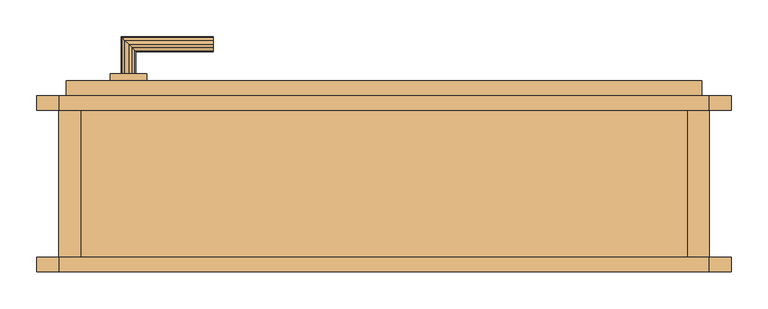
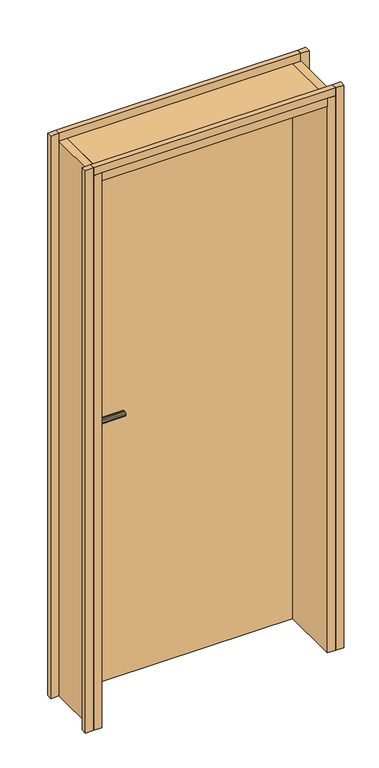
"""IFC4 building model written with IfcOpenShell, lengths in millimetres: door geometry, Tür."""

import ifcopenshell
import ifcopenshell.guid

model = None  # the IFC model being written
_history = None  # IfcOwnerHistory: only IFC2X3 demands one
_inside = {}  # id of a spatial element -> (the spatial element, [elements in it])
_under = {}  # id of a project, library or spatial element -> (it, [spatial elements below it])
_declared = {}  # id of a project -> (the project, [libraries it declares])
_typed = {}  # id of a type object -> (the type object, [elements of that type])
_made_of = {}  # id of a material, layer set ... -> (it, [elements and type objects made of it])


def new_model(schema):
    """Start an empty IFC model of exactly this schema.

    Asked for "IFC4X3", IfcOpenShell would pick the latest addendum, in which some entities
    have other attributes; the version numbers below select the first issue.
    IFC2X3 requires an IfcOwnerHistory on every rooted entity: one is made here for all.
    """
    global model, _history
    if schema == "IFC4X3":
        model = ifcopenshell.file(schema_version=(4, 3, 0, 0))
    else:
        model = ifcopenshell.file(schema=schema)
    _inside.clear()
    _under.clear()
    _declared.clear()
    _typed.clear()
    _made_of.clear()
    _history = None
    if model.schema == "IFC2X3":
        org = make("IfcOrganization", Name="unknown")
        user = make(
            "IfcPersonAndOrganization",
            ThePerson=make("IfcPerson", FamilyName="unknown"),
            TheOrganization=org,
        )
        app = make(
            "IfcApplication",
            ApplicationDeveloper=org,
            Version="unknown",
            ApplicationFullName="unknown",
            ApplicationIdentifier="unknown",
        )
        _history = make(
            "IfcOwnerHistory",
            OwningUser=user,
            OwningApplication=app,
            ChangeAction="ADDED",
            CreationDate=0,
        )
    return model


def make(cls, **values):
    """One entity of the class cls with the attributes given. An attribute that is None is left unset."""
    return model.create_entity(
        cls, **{name: value for name, value in values.items() if value is not None}
    )


def rooted(cls, **values):
    """An entity with a GlobalId (a new one), such as an element, a storey or a relation."""
    return make(cls, GlobalId=ifcopenshell.guid.new(), OwnerHistory=_history, **values)


def si_unit(unit_type, name, prefix=None):
    """IfcSIUnit, for example si_unit("LENGTHUNIT", "METRE", prefix="MILLI")."""
    return make("IfcSIUnit", UnitType=unit_type, Prefix=prefix, Name=name)


def assignment(units):
    """IfcUnitAssignment: the units of a project."""
    return None if units is None else make("IfcUnitAssignment", Units=units)


def point(xyz):
    """IfcCartesianPoint."""
    return None if xyz is None else make("IfcCartesianPoint", Coordinates=xyz)


def direction(xyz):
    """IfcDirection."""
    return None if xyz is None else make("IfcDirection", DirectionRatios=xyz)


def frame(location, z_axis=None, x_axis=None):
    """IfcAxis2Placement3D, a coordinate frame: its origin and axes. An axis left out is left unset."""
    return make(
        "IfcAxis2Placement3D",
        Location=point(location),
        Axis=direction(z_axis),
        RefDirection=direction(x_axis),
    )


def origin():
    """The frame at (0, 0, 0) with its axes left unset."""
    return frame((0.0, 0.0, 0.0))


def place(relative_to, where):
    """IfcLocalPlacement: puts the frame where relative to a parent placement (None: the world)."""
    return make(
        "IfcLocalPlacement", PlacementRelTo=relative_to, RelativePlacement=where
    )


def context(
    kind, dimensions, precision=None, world=None, true_north=None, identifier=None
):
    """IfcGeometricRepresentationContext, for example the 3D "Model" context."""
    return make(
        "IfcGeometricRepresentationContext",
        ContextIdentifier=identifier,
        ContextType=kind,
        CoordinateSpaceDimension=dimensions,
        Precision=precision,
        WorldCoordinateSystem=world,
        TrueNorth=true_north,
    )


def project(units=None, contexts=None):
    """IfcProject with its units and contexts."""
    return rooted(
        "IfcProject",
        Name="project",
        RepresentationContexts=contexts,
        UnitsInContext=assignment(units),
    )


def spatial(cls, under=None, at=None, **own):
    """A site, building, storey or space (cls), placed at a placement, below another one or the project."""
    s = rooted(cls, ObjectPlacement=at, **own)
    if under is not None:
        _under.setdefault(under.id(), (under, []))[1].append(s)
    return s


def polyline(points):
    """IfcPolyline through the points."""
    return make("IfcPolyline", Points=[point(p) for p in points])


def outline(outer, holes=None, kind="AREA"):
    """IfcArbitraryClosedProfileDef: a profile drawn as a closed curve; with holes, ...WithVoids."""
    if holes is None:
        return make("IfcArbitraryClosedProfileDef", ProfileType=kind, OuterCurve=outer)
    return make(
        "IfcArbitraryProfileDefWithVoids",
        ProfileType=kind,
        OuterCurve=outer,
        InnerCurves=holes,
    )


def extrude(swept, where, along, depth):
    """IfcExtrudedAreaSolid: the profile swept, set in the frame where, extruded along a direction by depth."""
    return make(
        "IfcExtrudedAreaSolid",
        SweptArea=swept,
        Position=where,
        ExtrudedDirection=direction(along),
        Depth=depth,
    )


def faces_of(points, faces, orient=None, outer=None):
    """IfcFace entities. A face is a list of loops; a loop is a list of indices into points, from 0.

    orient and outer hold one flag for each loop. By default every Orientation is true, the
    first loop of a face is its IfcFaceOuterBound and the others are IfcFaceBound.
    """
    made = []
    for i, loops in enumerate(faces):
        bounds = []
        for j, loop in enumerate(loops):
            is_outer = j == 0 if outer is None else outer[i][j]
            bounds.append(
                make(
                    "IfcFaceOuterBound" if is_outer else "IfcFaceBound",
                    Bound=make("IfcPolyLoop", Polygon=[points[k] for k in loop]),
                    Orientation=True if orient is None else orient[i][j],
                )
            )
        made.append(make("IfcFace", Bounds=bounds))
    return made


def faceted_brep(points, faces, orient=None, outer=None, voids=None):
    """IfcFacetedBrep: a solid bounded by flat faces; with voids (closed shells), ...WithVoids."""
    shared = [point(p) for p in points]
    hull = make("IfcClosedShell", CfsFaces=faces_of(shared, faces, orient, outer))
    if voids is None:
        return make("IfcFacetedBrep", Outer=hull)
    return make(
        "IfcFacetedBrepWithVoids",
        Outer=hull,
        Voids=[
            make(cls, CfsFaces=faces_of(shared, fs, o, b)) for cls, fs, o, b in voids
        ],
    )


def shape(context_of_items, identifier, shape_type, items):
    """IfcShapeRepresentation: the items that make up one representation, for example the "Body"."""
    return make(
        "IfcShapeRepresentation",
        ContextOfItems=context_of_items,
        RepresentationIdentifier=identifier,
        RepresentationType=shape_type,
        Items=items,
    )


def source(mapping_origin, context_of_items, identifier, shape_type, items):
    """IfcRepresentationMap: a shape defined once, which mapped items show again and again."""
    return make(
        "IfcRepresentationMap",
        MappingOrigin=mapping_origin,
        MappedRepresentation=shape(context_of_items, identifier, shape_type, items),
    )


def transform(
    local_origin,
    x_axis=None,
    y_axis=None,
    z_axis=None,
    scale=None,
    scale2=None,
    scale3=None,
    uniform=True,
):
    """IfcCartesianTransformationOperator3D, or its non-uniform kind. x_axis, y_axis, z_axis: its Axis1, 2, 3."""
    if uniform:
        return make(
            "IfcCartesianTransformationOperator3D",
            Axis1=direction(x_axis),
            Axis2=direction(y_axis),
            LocalOrigin=point(local_origin),
            Scale=scale,
            Axis3=direction(z_axis),
        )
    return make(
        "IfcCartesianTransformationOperator3DnonUniform",
        Axis1=direction(x_axis),
        Axis2=direction(y_axis),
        LocalOrigin=point(local_origin),
        Scale=scale,
        Axis3=direction(z_axis),
        Scale2=scale2,
        Scale3=scale3,
    )


def mapped(mapping_source, mapping_target):
    """IfcMappedItem: shows the shape of a source again, moved by a transform."""
    return make(
        "IfcMappedItem", MappingSource=mapping_source, MappingTarget=mapping_target
    )


def made_of(thing, what):
    """Note that an element or type object is made of a material, layer set ...; save() writes the relation."""
    if what is not None:
        _made_of.setdefault(what.id(), (what, []))[1].append(thing)
    return thing


def element(
    cls,
    number,
    at=None,
    inside=None,
    cuts=None,
    type_object=None,
    material=None,
    context=None,
    identifier="Body",
    shape_type=None,
    held_by="IfcProductDefinitionShape",
    body=None,
    shapes=None,
    **own,
):
    """One element of the class cls, such as IfcWall. Its Tag is "e" and its number.

    at: its placement. inside: the storey or other place that contains it. cuts: it is an
    opening in that element (IfcRelVoidsElement). A single representation is given by context,
    identifier, shape_type and body (its items); several are given by shapes. held_by: the class
    of the entity that holds the representations. save() writes the other relations.
    """
    e = rooted(cls, Tag="e%d" % number, ObjectPlacement=at, **own)
    if body is not None:
        shapes = [shape(context, identifier, shape_type, body)]
    if shapes is not None:
        e.Representation = make(held_by, Representations=shapes)
    if inside is not None:
        _inside.setdefault(inside.id(), (inside, []))[1].append(e)
    if cuts is not None:
        rooted(
            "IfcRelVoidsElement", RelatingBuildingElement=cuts, RelatedOpeningElement=e
        )
    if type_object is not None:
        _typed.setdefault(type_object.id(), (type_object, []))[1].append(e)
    return made_of(e, material)


def aggregate(whole, parts):
    """IfcRelAggregates: a whole, such as a stair, and the parts it consists of."""
    return rooted("IfcRelAggregates", RelatingObject=whole, RelatedObjects=parts)


def save(model, path):
    """Write the relations noted so far, then the file.

    IfcRelAggregates (storeys below a building ...), IfcRelContainedInSpatialStructure (elements
    in a storey), IfcRelDefinesByType, IfcRelAssociatesMaterial and IfcRelDeclares: one each for
    every whole, place, type object, material and project.
    """
    for whole, parts in _under.values():
        aggregate(whole, parts)
    for where, things in _inside.values():
        rooted(
            "IfcRelContainedInSpatialStructure",
            RelatedElements=things,
            RelatingStructure=where,
        )
    for kind, things in _typed.values():
        rooted("IfcRelDefinesByType", RelatedObjects=things, RelatingType=kind)
    for what, things in _made_of.values():
        rooted("IfcRelAssociatesMaterial", RelatedObjects=things, RelatingMaterial=what)
    for by, libraries in _declared.values():
        rooted("IfcRelDeclares", RelatingContext=by, RelatedDefinitions=libraries)
    model.write(path)


def door_56521e71(model_context):
    return source(origin(), model_context, "Body", "SolidModel", [
        extrude(outline(polyline([(915.0, 220.0), (915.0, 200.0), (885.0, 200.0), (885.0, 220.0), (915.0, 220.0)])), frame((0.0, 0.0, 140.0), z_axis=(0.0, 0.0, 1.0), x_axis=(1.0, 0.0, 0.0)), (0.0, 0.0, 1.0), 2175.0),
        extrude(outline(polyline([(120.0, 240.0), (70.0, 240.0), (70.0, 250.0), (120.0, 250.0), (120.0, 240.0)])), frame((0.0, 0.0, 1050.0), z_axis=(0.0, 0.0, 1.0), x_axis=(1.0, 0.0, 0.0)), (0.0, 0.0, 1.0), 215.0),
        extrude(outline(polyline([(915.0, 0.0), (915.0, -20.0), (885.0, -20.0), (885.0, 0.0), (915.0, 0.0)])), frame((0.0, 0.0, 140.0), z_axis=(0.0, 0.0, 1.0), x_axis=(1.0, 0.0, 0.0)), (0.0, 0.0, 1.0), 2175.0),
        faceted_brep([(90.0, 190.0, 1198.660254), (95.0, 190.0, 1200.0), (100.0, 190.0, 1198.660254), (103.660254, 190.0, 1195.0), (105.0, 190.0, 1190.0), (103.660254, 190.0, 1185.0), (100.0, 190.0, 1181.339746), (95.0, 190.0, 1180.0), (90.0, 190.0, 1181.339746), (86.339746, 190.0, 1185.0), (85.0, 190.0, 1190.0), (86.339746, 190.0, 1195.0), (95.0, 150.0, 1200.0), (90.0, 145.0, 1198.660254), (86.339746, 141.339746, 1195.0), (85.0, 140.0, 1190.0), (86.339746, 141.339746, 1185.0), (90.0, 145.0, 1181.339746), (95.0, 150.0, 1180.0), (100.0, 155.0, 1181.339746), (103.660254, 158.660254, 1185.0), (105.0, 160.0, 1190.0), (103.660254, 158.660254, 1195.0), (100.0, 155.0, 1198.660254), (210.0, 155.0, 1198.660254), (210.0, 150.0, 1200.0), (210.0, 145.0, 1198.660254), (210.0, 141.339746, 1195.0), (210.0, 140.0, 1190.0), (210.0, 141.339746, 1185.0), (210.0, 145.0, 1181.339746), (210.0, 150.0, 1180.0), (210.0, 155.0, 1181.339746), (210.0, 158.660254, 1185.0), (210.0, 160.0, 1190.0), (210.0, 158.660254, 1195.0)], [[[0, 1, 2, 3, 4, 5, 6, 7, 8, 9, 10, 11]], [[12, 1, 0, 13]], [[13, 0, 11, 14]], [[14, 11, 10, 15]], [[15, 10, 9, 16]], [[16, 9, 8, 17]], [[17, 8, 7, 18]], [[18, 7, 6, 19]], [[19, 6, 5, 20]], [[20, 5, 4, 21]], [[21, 4, 3, 22]], [[22, 3, 2, 23]], [[23, 2, 1, 12]], [[24, 25, 26, 27, 28, 29, 30, 31, 32, 33, 34, 35]], [[25, 12, 13, 26]], [[26, 13, 14, 27]], [[27, 14, 15, 28]], [[28, 15, 16, 29]], [[29, 16, 17, 30]], [[30, 17, 18, 31]], [[31, 18, 19, 32]], [[32, 19, 20, 33]], [[33, 20, 21, 34]], [[34, 21, 22, 35]], [[35, 22, 23, 24]], [[24, 23, 12, 25]]]),
        extrude(outline(polyline([(30.0, -20.0), (0.0, -20.0), (0.0, 220.0), (30.0, 220.0), (30.0, -20.0)])), frame((0.0, 0.0, 140.0), z_axis=(0.0, 0.0, 1.0), x_axis=(1.0, 0.0, 0.0)), (0.0, 0.0, 1.0), 2145.0),
        extrude(outline(polyline([(70.0, 190.0), (70.0, 200.0), (120.0, 200.0), (120.0, 190.0), (70.0, 190.0)])), frame((0.0, 0.0, 1050.0), z_axis=(0.0, 0.0, 1.0), x_axis=(1.0, 0.0, 0.0)), (0.0, 0.0, 1.0), 215.0),
        extrude(outline(polyline([(0.0, 200.0), (-30.0, 200.0), (-30.0, 220.0), (0.0, 220.0), (0.0, 200.0)])), frame((0.0, 0.0, 140.0), z_axis=(0.0, 0.0, 1.0), x_axis=(1.0, 0.0, 0.0)), (0.0, 0.0, 1.0), 2175.0),
        extrude(outline(polyline([(855.0, -20.0), (30.0, -20.0), (30.0, 220.0), (855.0, 220.0), (855.0, -20.0)])), frame((0.0, 0.0, 2255.0), z_axis=(0.0, 0.0, 1.0), x_axis=(1.0, 0.0, 0.0)), (0.0, 0.0, 1.0), 30.0),
        extrude(outline(polyline([(875.0, 200.0), (10.0, 200.0), (10.0, 240.0), (875.0, 240.0), (875.0, 200.0)])), frame((0.0, 0.0, 140.0), z_axis=(0.0, 0.0, 1.0), x_axis=(1.0, 0.0, 0.0)), (0.0, 0.0, 1.0), 2135.0),
        extrude(outline(polyline([(0.0, -20.0), (-30.0, -20.0), (-30.0, 0.0), (0.0, 0.0), (0.0, -20.0)])), frame((0.0, 0.0, 140.0), z_axis=(0.0, 0.0, 1.0), x_axis=(1.0, 0.0, 0.0)), (0.0, 0.0, 1.0), 2175.0),
        extrude(outline(polyline([(885.0, 200.0), (0.0, 200.0), (0.0, 220.0), (885.0, 220.0), (885.0, 200.0)])), frame((0.0, 0.0, 2285.0), z_axis=(0.0, 0.0, 1.0), x_axis=(1.0, 0.0, 0.0)), (0.0, 0.0, 1.0), 30.0),
        extrude(outline(polyline([(885.0, -20.0), (855.0, -20.0), (855.0, 220.0), (885.0, 220.0), (885.0, -20.0)])), frame((0.0, 0.0, 140.0), z_axis=(0.0, 0.0, 1.0), x_axis=(1.0, 0.0, 0.0)), (0.0, 0.0, 1.0), 2145.0),
        extrude(outline(polyline([(885.0, -20.0), (0.0, -20.0), (0.0, 0.0), (885.0, 0.0), (885.0, -20.0)])), frame((0.0, 0.0, 2285.0), z_axis=(0.0, 0.0, 1.0), x_axis=(1.0, 0.0, 0.0)), (0.0, 0.0, 1.0), 30.0),
        faceted_brep([(100.0, 250.0, 1198.660254), (95.0, 250.0, 1200.0), (90.0, 250.0, 1198.660254), (86.339746, 250.0, 1195.0), (85.0, 250.0, 1190.0), (86.339746, 250.0, 1185.0), (90.0, 250.0, 1181.339746), (95.0, 250.0, 1180.0), (100.0, 250.0, 1181.339746), (103.660254, 250.0, 1185.0), (105.0, 250.0, 1190.0), (103.660254, 250.0, 1195.0), (95.0, 290.0, 1200.0), (90.0, 295.0, 1198.660254), (86.339746, 298.660254, 1195.0), (85.0, 300.0, 1190.0), (86.339746, 298.660254, 1185.0), (90.0, 295.0, 1181.339746), (95.0, 290.0, 1180.0), (100.0, 285.0, 1181.339746), (103.660254, 281.339746, 1185.0), (105.0, 280.0, 1190.0), (103.660254, 281.339746, 1195.0), (100.0, 285.0, 1198.660254), (210.0, 295.0, 1198.660254), (210.0, 290.0, 1200.0), (210.0, 285.0, 1198.660254), (210.0, 281.339746, 1195.0), (210.0, 280.0, 1190.0), (210.0, 281.339746, 1185.0), (210.0, 285.0, 1181.339746), (210.0, 290.0, 1180.0), (210.0, 295.0, 1181.339746), (210.0, 298.660254, 1185.0), (210.0, 300.0, 1190.0), (210.0, 298.660254, 1195.0)], [[[0, 1, 2, 3, 4, 5, 6, 7, 8, 9, 10, 11]], [[2, 1, 12, 13]], [[3, 2, 13, 14]], [[4, 3, 14, 15]], [[5, 4, 15, 16]], [[6, 5, 16, 17]], [[7, 6, 17, 18]], [[8, 7, 18, 19]], [[9, 8, 19, 20]], [[10, 9, 20, 21]], [[11, 10, 21, 22]], [[0, 11, 22, 23]], [[1, 0, 23, 12]], [[24, 25, 26, 27, 28, 29, 30, 31, 32, 33, 34, 35]], [[13, 12, 25, 24]], [[14, 13, 24, 35]], [[15, 14, 35, 34]], [[16, 15, 34, 33]], [[17, 16, 33, 32]], [[18, 17, 32, 31]], [[19, 18, 31, 30]], [[20, 19, 30, 29]], [[21, 20, 29, 28]], [[22, 21, 28, 27]], [[23, 22, 27, 26]], [[12, 23, 26, 25]]]),
    ])


if __name__ == "__main__":
    model = new_model("IFC4")
    model_context = context("Model", 3, world=origin())
    ifc_project = project(units=[si_unit("LENGTHUNIT", "METRE", prefix="MILLI")], contexts=[model_context])
    site = spatial("IfcSite", under=ifc_project)
    building = spatial("IfcBuilding", under=site)
    placement = place(None, origin())
    door_shape = door_56521e71(model_context)
    element("IfcDoor", 1, ObjectType="Tür", at=placement, inside=building, context=model_context, shape_type="MappedRepresentation", body=[
        mapped(door_shape, transform((0.0, 0.0, 0.0), x_axis=(1.0, 0.0, 0.0), y_axis=(0.0, 1.0, 0.0), z_axis=(0.0, 0.0, 1.0))),
    ])
    save(model, "model.ifc")

# Revit data of these elements
# Type "Tür"
#   Type Mark = "29"
# Element 1 (IfcDoor, "Tür")
#   Materials on its faces: "tuer_beschlag", "tuer_holzzarge"
# Materials
#   "tuer_beschlag": class "Unassigned", colour RGB 128 128 128, transparency 0
#   "tuer_holzzarge": class "Unassigned", colour RGB 255 255 255, transparency 0
